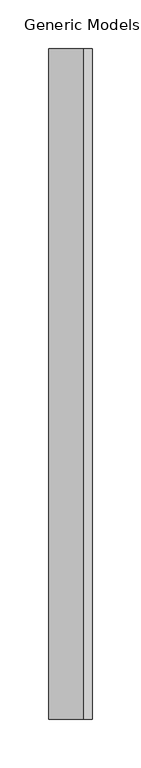
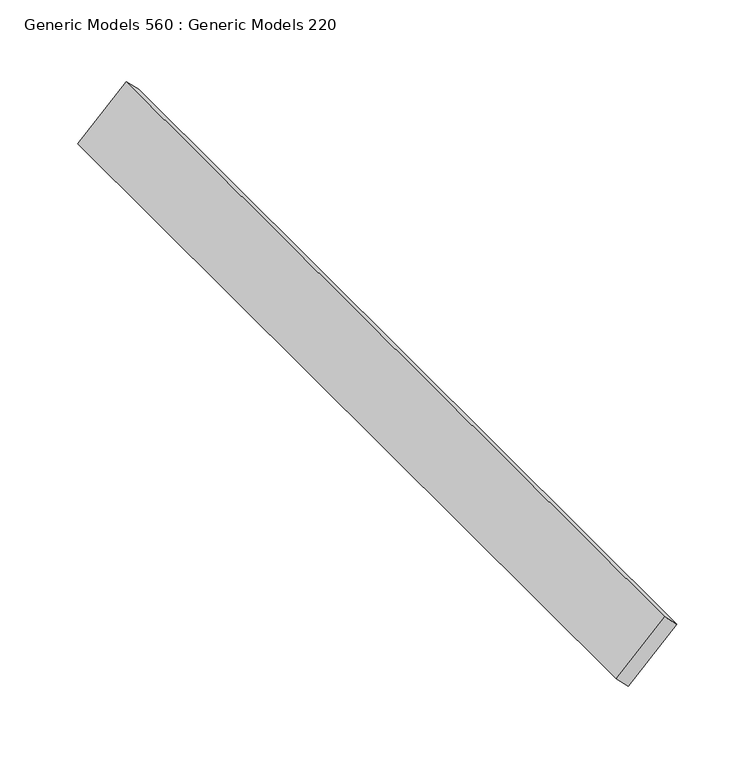
"""IFC4 building model written with IfcOpenShell, lengths in millimetres: proxy geometry, Generic Models 560 : Generic Models 220."""

from ifc_helpers import new_model, si_unit, frame, origin, place, context, project, spatial, polyline, outline, extrude, source, transform, mapped, element, save


def generic_models_560_generic_models_220_3b74700a(model_context):
    return source(origin(), model_context, "Body", "SweptSolid", [
        extrude(outline(polyline([(0.0, -12.7000001), (0.0, 0.0), (690.8142348, 0.0), (690.8142348, -12.7000001), (0.0, -12.7000001)])), frame((7841.3059863, 4539.4872686, 124366.6399101), z_axis=(0.7071067811868034, 0.0, 0.7071067811862918), x_axis=(0.0, -1.0, 0.0)), (0.0, 0.0, 1.0), 50.8),
    ])


if __name__ == "__main__":
    model = new_model("IFC4")
    model_context = context("Model", 3, world=origin())
    ifc_project = project(units=[si_unit("LENGTHUNIT", "METRE", prefix="MILLI")], contexts=[model_context])
    site = spatial("IfcSite", under=ifc_project)
    building = spatial("IfcBuilding", under=site)
    placement = place(None, origin())
    generic_models_560_generic_models_220_shape = generic_models_560_generic_models_220_3b74700a(model_context)
    element("IfcBuildingElementProxy", 1, Name="Generic Models 560 : Generic Models 220", ObjectType="Generic Models 560 : Generic Models 220", at=placement, inside=building, context=model_context, shape_type="MappedRepresentation", body=[
        mapped(generic_models_560_generic_models_220_shape, transform((0.0, 0.0, 0.0), x_axis=(1.0, 0.0, 0.0), y_axis=(0.0, 1.0, 0.0), z_axis=(0.0, 0.0, 1.0))),
    ])
    save(model, "model.ifc")

# Revit data of these elements
# Element 1 (IfcBuildingElementProxy, "Generic Models 560 : Generic Models 220")
#   Materials on its faces: "_WOOD TONE ALUMINUM EXTRUSION SLAT BY KNOTWOOD"
# Materials
#   "_WOOD TONE ALUMINUM EXTRUSION SLAT BY KNOTWOOD": class "Generic", colour RGB 177 130 114, transparency 0, Cost = 0
